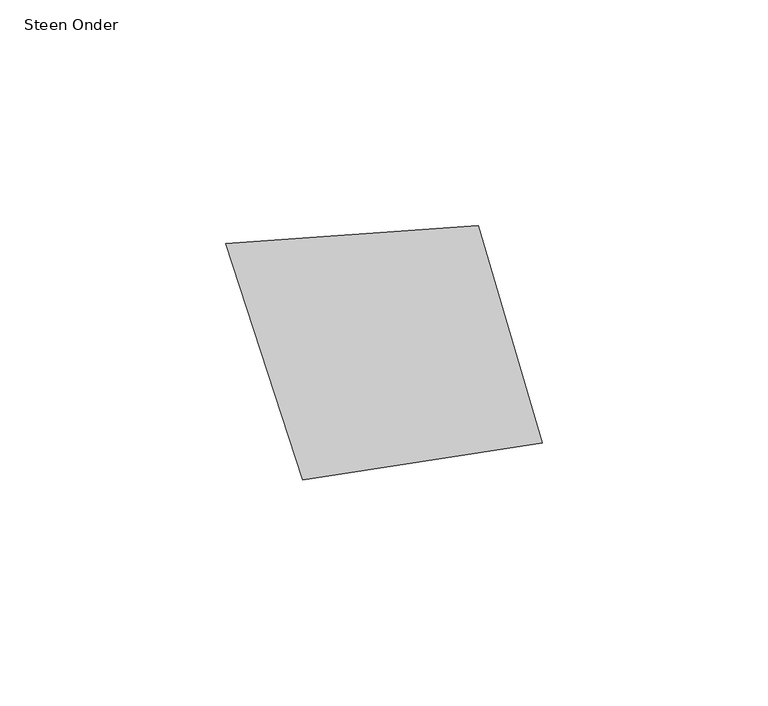
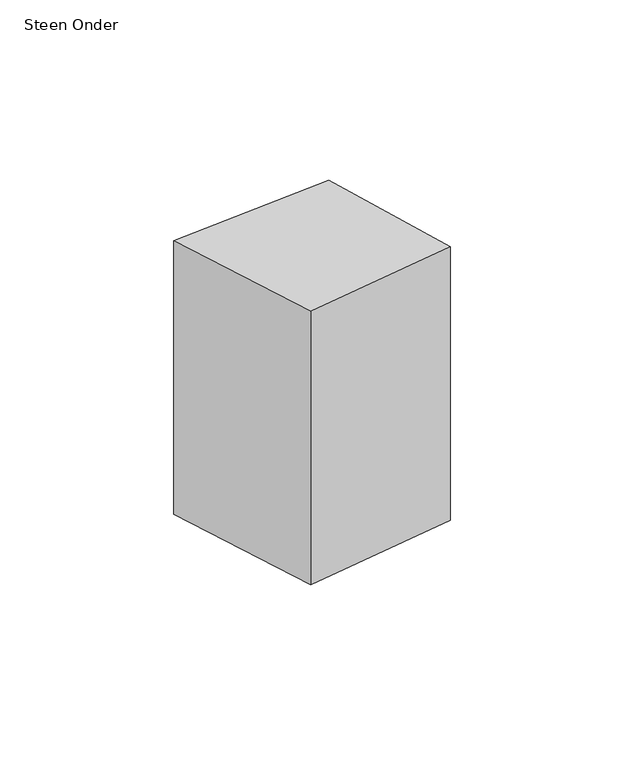
"""IFC4 building model written with IfcOpenShell, lengths in millimetres: proxy geometry, 00_GMA_steen_versie_4 : Steen Onder."""

from ifc_helpers import new_model, si_unit, origin, origin_with_axes, place, context, project, spatial, polyline, outline, extrude, source, transform, mapped, element, save


def steen_onder_470f7271(model_context):
    return source(origin(), model_context, "Body", "SweptSolid", [
        extrude(outline(polyline([(94.1726884, 89.9316428), (108.3739221, 41.68389), (55.2698309, 33.4714181), (38.160247, 85.8970334), (94.1726884, 89.9316428)])), origin_with_axes(), (0.0, 0.0, 1.0), 100.0),
    ])


if __name__ == "__main__":
    model = new_model("IFC4")
    model_context = context("Model", 3, world=origin())
    ifc_project = project(units=[si_unit("LENGTHUNIT", "METRE", prefix="MILLI")], contexts=[model_context])
    site = spatial("IfcSite", under=ifc_project)
    building = spatial("IfcBuilding", under=site)
    placement = place(None, origin())
    steen_onder_shape = steen_onder_470f7271(model_context)
    element("IfcBuildingElementProxy", 1, Name="00_GMA_steen_versie_4 : Steen Onder", ObjectType="00_GMA_steen_versie_4 : Steen Onder", at=placement, inside=building, context=model_context, shape_type="MappedRepresentation", body=[
        mapped(steen_onder_shape, transform((0.0, 0.0, 0.0), x_axis=(1.0, 0.0, 0.0), y_axis=(0.0, 1.0, 0.0), z_axis=(0.0, 0.0, 1.0))),
    ])
    save(model, "model.ifc")

# Revit data of these elements
# Type "00_GMA_steen_versie_4 : Steen Onder"
#   StootVoegHalfBoven [instance default] = 5 mm
#   StootVoegHalf [instance default] = 5 mm
#   StootVoegBreedteOnder = 10 mm
#   StootVoegBreedteBoven = 10 mm
#   Steendikte = 100 mm
#   LintVoegOnderHalf = 0 mm
#   LintVoegOnder = 0 mm
#   LintVoegBovenHalf = 5 mm
#   LintVoegBoven = 10 mm
#   materiaal = none
#   MateriaalVoeg = none
#   Default Elevation = 0
